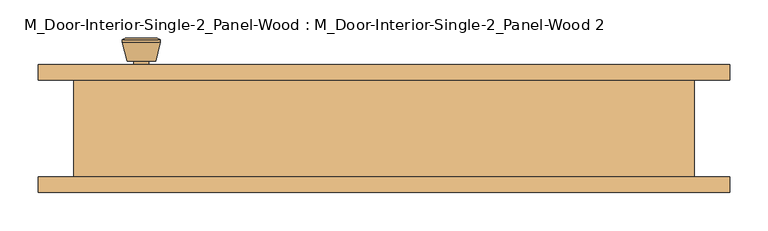
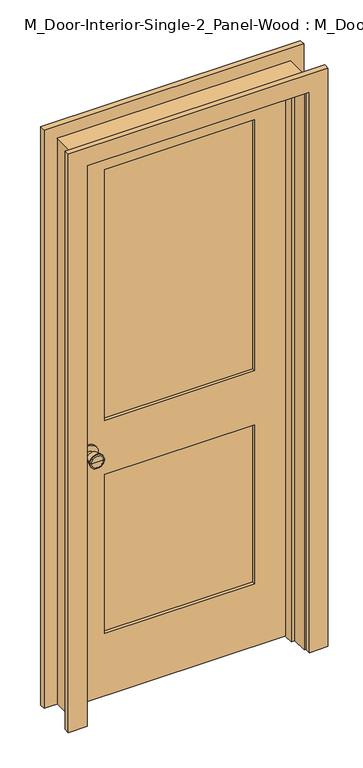
"""IFC4 building model written with IfcOpenShell, lengths in millimetres: door geometry, M_Door-Interior-Single-2_Panel-Wood : M_Door-Interior-Single-2_Panel-Wood 2."""

from ifc_helpers import new_model, si_unit, point, frame, frame_2d, origin, place, context, project, spatial, polyline, circle_curve, trimmed, segment, composite_curve, outline, extrude, faceted_brep, source, transform, mapped, element, save
from ifc_brep_helpers import plane_surface, cylinder_surface, revolved_surface, advanced_brep


def m_door_interior_single_2_panel_wood_m_door_interior_single_2_3351e8e6(model_context):
    return source(origin(), model_context, "Body", "SolidModel", [
        advanced_brep(
        [(-317.5, 19.325, 914.4), (-307.5, 19.325, 914.4), (-327.5, 19.325, 914.4), (-297.0241324, -29.675, 914.4), (-317.5, -29.675, 914.4), (-337.9758676, -29.675, 914.4), (-292.5, -27.8471319, 914.4), (-342.5, -27.8471319, 914.4), (-292.5, -24.3834537, 914.4), (-342.5, -24.3834537, 914.4), (-298.863764, 0.325, 914.4), (-336.136236, 0.325, 914.4), (-307.5, 0.325, 914.4), (-327.5, 0.325, 914.4)],
        [
            (0, 1),
            (1, 2, circle_curve(frame((-317.5, 19.325, 914.4), z_axis=(0.0, 1.0, 0.0), x_axis=(-1.0, 0.0, 0.0)), 10.0)),
            (2, 0),
            (2, 1, circle_curve(frame((-317.5, 19.325, 914.4), z_axis=(0.0, 1.0, 0.0), x_axis=(-1.0, 0.0, 0.0)), 10.0)),
            (3, 4),
            (4, 5),
            (5, 3, circle_curve(frame((-317.5, -29.675, 914.4), z_axis=(0.0, -1.0, 0.0), x_axis=(-1.0, 0.0, 0.0)), 20.4758676)),
            (3, 5, circle_curve(frame((-317.5, -29.675, 914.4), z_axis=(0.0, -1.0, 0.0), x_axis=(-1.0, 0.0, 0.0)), 20.4758676)),
            (6, 3),
            (5, 7),
            (7, 6, circle_curve(frame((-317.5, -27.8471319, 914.4), z_axis=(0.0, -1.0, 0.0), x_axis=(-1.0, 0.0, 0.0)), 25.0)),
            (6, 7, circle_curve(frame((-317.5, -27.8471319, 914.4), z_axis=(0.0, -1.0, 0.0), x_axis=(-1.0, 0.0, 0.0)), 25.0)),
            (8, 6),
            (7, 9),
            (9, 8, circle_curve(frame((-317.5, -24.3834537, 914.4), z_axis=(0.0, -1.0, 0.0), x_axis=(-1.0, 0.0, 0.0)), 25.0)),
            (8, 9, circle_curve(frame((-317.5, -24.3834537, 914.4), z_axis=(0.0, -1.0, 0.0), x_axis=(-1.0, 0.0, 0.0)), 25.0)),
            (10, 8),
            (9, 11),
            (11, 10, circle_curve(frame((-317.5, 0.325, 914.4), z_axis=(0.0, -1.0, 0.0), x_axis=(-1.0, 0.0, 0.0)), 18.636236)),
            (10, 11, circle_curve(frame((-317.5, 0.325, 914.4), z_axis=(0.0, -1.0, 0.0), x_axis=(-1.0, 0.0, 0.0)), 18.636236)),
            (12, 10),
            (11, 13),
            (13, 12, circle_curve(frame((-317.5, 0.325, 914.4), z_axis=(0.0, -1.0, 0.0), x_axis=(-1.0, 0.0, 0.0)), 10.0)),
            (12, 13, circle_curve(frame((-317.5, 0.325, 914.4), z_axis=(0.0, -1.0, 0.0), x_axis=(-1.0, 0.0, 0.0)), 10.0)),
            (1, 12),
            (13, 2),
        ],
        [
            plane_surface(frame((-317.5, 19.325, 914.4), z_axis=(0.0, 1.0, 0.0), x_axis=(-1.0, 0.0, 0.0))),
            plane_surface(frame((-317.5, -29.675, 914.4), z_axis=(0.0, -1.0, 0.0), x_axis=(-1.0, 0.0, 0.0))),
            revolved_surface(polyline([(-337.9758676, -29.675, 914.4), (-342.5, -27.8471319, 914.4)]), (-317.5, 19.325, 914.4), (0.0, 1.0, 0.0)),
            cylinder_surface(frame((-317.5, 19.325, 914.4), z_axis=(0.0, 1.0, 0.0), x_axis=(-1.0, 0.0, 0.0)), 25.0),
            revolved_surface(polyline([(-342.5, -24.3834537, 914.4), (-336.136236, 0.325, 914.4)]), (-317.5, 19.325, 914.4), (0.0, 1.0, 0.0)),
            plane_surface(frame((-317.5, 0.325, 914.4), z_axis=(0.0, 1.0, 0.0), x_axis=(-1.0, 0.0, 0.0))),
            cylinder_surface(frame((-317.5, 19.325, 914.4), z_axis=(0.0, 1.0, 0.0), x_axis=(-1.0, 0.0, 0.0)), 10.0),
        ],
        [
            (0, [[1, 2, 3]]),
            (0, [[-3, 4, -1]]),
            (1, [[5, 6, 7]]),
            (1, [[-6, -5, 8]]),
            (2, [[9, -7, 10, 11]]),
            (2, [[-10, -8, -9, 12]]),
            (3, [[13, -11, 14, 15]]),
            (3, [[-14, -12, -13, 16]]),
            (4, [[17, -15, 18, 19]]),
            (4, [[-18, -16, -17, 20]]),
            (5, [[21, -19, 22, 23]]),
            (5, [[-22, -20, -21, 24]]),
            (6, [[25, -23, 26, -2]]),
            (6, [[-26, -24, -25, -4]]),
        ],
    ),
        extrude(outline(composite_curve([segment(trimmed(circle_curve(frame_2d((914.4, -317.5)), 30.0), [point((914.4, -347.5))], [point((914.4, -287.5))], False, "CARTESIAN"), True, "CONTINUOUS"), segment(trimmed(circle_curve(frame_2d((914.4, -317.5)), 30.0), [point((914.4, -287.5))], [point((914.4, -347.5))], False, "CARTESIAN"), True, "CONTINUOUS")], self_intersect=False)), frame((0.0, 19.325, 0.0), z_axis=(0.0, 1.0, 0.0), x_axis=(0.0, 0.0, 1.0)), (0.0, 0.0, 1.0), 6.0),
        advanced_brep(
        [(-317.5, 66.325, 914.4), (-327.5, 66.325, 914.4), (-307.5, 66.325, 914.4), (-297.0241324, 115.325, 914.4), (-337.9758676, 115.325, 914.4), (-317.5, 115.325, 914.4), (-292.5, 113.4971319, 914.4), (-342.5, 113.4971319, 914.4), (-292.5, 110.0334537, 914.4), (-342.5, 110.0334537, 914.4), (-298.863764, 85.325, 914.4), (-336.136236, 85.325, 914.4), (-307.5, 85.325, 914.4), (-327.5, 85.325, 914.4)],
        [
            (0, 1),
            (1, 2, circle_curve(frame((-317.5, 66.325, 914.4), z_axis=(0.0, -1.0, 0.0), x_axis=(-1.0, 0.0, 0.0)), 10.0)),
            (2, 0),
            (2, 1, circle_curve(frame((-317.5, 66.325, 914.4), z_axis=(0.0, -1.0, 0.0), x_axis=(-1.0, 0.0, 0.0)), 10.0)),
            (3, 4, circle_curve(frame((-317.5, 115.325, 914.4), z_axis=(0.0, 1.0, 0.0), x_axis=(-1.0, 0.0, 0.0)), 20.4758676)),
            (4, 5),
            (5, 3),
            (4, 3, circle_curve(frame((-317.5, 115.325, 914.4), z_axis=(0.0, 1.0, 0.0), x_axis=(-1.0, 0.0, 0.0)), 20.4758676)),
            (6, 7, circle_curve(frame((-317.5, 113.4971319, 914.4), z_axis=(0.0, 1.0, 0.0), x_axis=(-1.0, 0.0, 0.0)), 25.0)),
            (7, 4),
            (3, 6),
            (7, 6, circle_curve(frame((-317.5, 113.4971319, 914.4), z_axis=(0.0, 1.0, 0.0), x_axis=(-1.0, 0.0, 0.0)), 25.0)),
            (8, 9, circle_curve(frame((-317.5, 110.0334537, 914.4), z_axis=(0.0, 1.0, 0.0), x_axis=(-1.0, 0.0, 0.0)), 25.0)),
            (9, 7),
            (6, 8),
            (9, 8, circle_curve(frame((-317.5, 110.0334537, 914.4), z_axis=(0.0, 1.0, 0.0), x_axis=(-1.0, 0.0, 0.0)), 25.0)),
            (10, 11, circle_curve(frame((-317.5, 85.325, 914.4), z_axis=(0.0, 1.0, 0.0), x_axis=(-1.0, 0.0, 0.0)), 18.636236)),
            (11, 9),
            (8, 10),
            (11, 10, circle_curve(frame((-317.5, 85.325, 914.4), z_axis=(0.0, 1.0, 0.0), x_axis=(-1.0, 0.0, 0.0)), 18.636236)),
            (12, 13, circle_curve(frame((-317.5, 85.325, 914.4), z_axis=(0.0, 1.0, 0.0), x_axis=(-1.0, 0.0, 0.0)), 10.0)),
            (13, 11),
            (10, 12),
            (13, 12, circle_curve(frame((-317.5, 85.325, 914.4), z_axis=(0.0, 1.0, 0.0), x_axis=(-1.0, 0.0, 0.0)), 10.0)),
            (1, 13),
            (12, 2),
        ],
        [
            plane_surface(frame((-317.5, 66.325, 914.4), z_axis=(0.0, -1.0, 0.0), x_axis=(-1.0, 0.0, 0.0))),
            plane_surface(frame((-317.5, 115.325, 914.4), z_axis=(0.0, 1.0, 0.0), x_axis=(-1.0, 0.0, 0.0))),
            revolved_surface(polyline([(-337.9758676, 115.325, 914.4), (-342.5, 113.4971319, 914.4)]), (-317.5, 66.325, 914.4), (0.0, -1.0, 0.0)),
            cylinder_surface(frame((-317.5, 66.325, 914.4), z_axis=(0.0, -1.0, 0.0), x_axis=(-1.0, 0.0, 0.0)), 25.0),
            revolved_surface(polyline([(-342.5, 110.0334537, 914.4), (-336.136236, 85.325, 914.4)]), (-317.5, 66.325, 914.4), (0.0, -1.0, 0.0)),
            plane_surface(frame((-317.5, 85.325, 914.4), z_axis=(0.0, -1.0, 0.0), x_axis=(-1.0, 0.0, 0.0))),
            cylinder_surface(frame((-317.5, 66.325, 914.4), z_axis=(0.0, -1.0, 0.0), x_axis=(-1.0, 0.0, 0.0)), 10.0),
        ],
        [
            (0, [[1, 2, 3]]),
            (0, [[-3, 4, -1]]),
            (1, [[5, 6, 7]]),
            (1, [[8, -7, -6]]),
            (2, [[9, 10, -5, 11]]),
            (2, [[12, -11, -8, -10]]),
            (3, [[13, 14, -9, 15]]),
            (3, [[16, -15, -12, -14]]),
            (4, [[17, 18, -13, 19]]),
            (4, [[20, -19, -16, -18]]),
            (5, [[21, 22, -17, 23]]),
            (5, [[24, -23, -20, -22]]),
            (6, [[-2, 25, -21, 26]]),
            (6, [[-4, -26, -24, -25]]),
        ],
    ),
        extrude(outline(composite_curve([segment(trimmed(circle_curve(frame_2d((914.4, -317.5)), 30.0), [point((914.4, -347.5))], [point((914.4, -287.5))], False, "CARTESIAN"), True, "CONTINUOUS"), segment(trimmed(circle_curve(frame_2d((914.4, -317.5)), 30.0), [point((914.4, -287.5))], [point((914.4, -347.5))], False, "CARTESIAN"), True, "CONTINUOUS")], self_intersect=False)), frame((0.0, 60.325, 0.0), z_axis=(0.0, 1.0, 0.0), x_axis=(0.0, 0.0, 1.0)), (0.0, 0.0, 1.0), 6.0),
        extrude(outline(polyline([(261.0, 36.9916667), (-261.0, 36.9916667), (-261.0, 48.6583333), (261.0, 48.6583333), (261.0, 36.9916667)])), frame((0.0, 0.0, 1014.4), z_axis=(0.0, 0.0, 1.0), x_axis=(1.0, 0.0, 0.0)), (0.0, 0.0, 1.0), 923.0),
        extrude(outline(polyline([(261.0, 36.9916667), (-261.0, 36.9916667), (-261.0, 48.6583333), (261.0, 48.6583333), (261.0, 36.9916667)])), frame((0.0, 0.0, 230.0), z_axis=(0.0, 0.0, 1.0), x_axis=(1.0, 0.0, 0.0)), (0.0, 0.0, 1.0), 584.4),
        extrude(outline(polyline([(2057.4, -381.0), (0.0, -381.0), (0.0, 381.0), (2057.4, 381.0), (2057.4, -381.0)]), holes=[polyline([(1937.4, -261.0), (1937.4, 261.0), (1014.4, 261.0), (1014.4, -261.0), (1937.4, -261.0)]), polyline([(814.4, -261.0), (814.4, 261.0), (230.0, 261.0), (230.0, -261.0), (814.4, -261.0)])]), frame((0.0, 25.325, 0.0), z_axis=(0.0, 1.0, 0.0), x_axis=(0.0, 0.0, 1.0)), (0.0, 0.0, 1.0), 35.0),
        faceted_brep([(406.0, 60.325, 0.0), (406.0, -66.675, 0.0), (381.0, -66.675, 0.0), (381.0, -9.6, 0.0), (368.3, -9.6, 0.0), (368.3, 25.325, 0.0), (381.0, 25.325, 0.0), (381.0, 60.325, 0.0), (406.0, 60.325, 2082.4), (406.0, -66.675, 2082.4), (-406.0, -66.675, 2082.4), (-406.0, -66.675, 0.0), (-381.0, -66.675, 0.0), (-381.0, -66.675, 2057.4), (381.0, -66.675, 2057.4), (381.0, -9.6, 2057.4), (-381.0, -9.6, 2057.4), (-381.0, -9.6, 0.0), (-368.3, -9.6, 0.0), (-368.3, -9.6, 2044.7), (368.3, -9.6, 2044.7), (368.3, 25.325, 2044.7), (-368.3, 25.325, 2044.7), (-368.3, 25.325, 0.0), (-381.0, 25.325, 0.0), (-381.0, 25.325, 2057.4), (381.0, 25.325, 2057.4), (381.0, 60.325, 2057.4), (-381.0, 60.325, 2057.4), (-381.0, 60.325, 0.0), (-406.0, 60.325, 0.0), (-406.0, 60.325, 2082.4)], [[[0, 1, 2, 3, 4, 5, 6, 7]], [[1, 0, 8, 9]], [[2, 1, 9, 10, 11, 12, 13, 14]], [[3, 2, 14, 15]], [[4, 3, 15, 16, 17, 18, 19, 20]], [[5, 4, 20, 21]], [[6, 5, 21, 22, 23, 24, 25, 26]], [[7, 6, 26, 27]], [[0, 7, 27, 28, 29, 30, 31, 8]], [[9, 8, 31, 10]], [[15, 14, 13, 16]], [[21, 20, 19, 22]], [[27, 26, 25, 28]], [[30, 29, 24, 23, 18, 17, 12, 11]], [[10, 31, 30, 11]], [[16, 13, 12, 17]], [[22, 19, 18, 23]], [[28, 25, 24, 29]]]),
        extrude(outline(polyline([(0.0, 387.35), (0.0, 452.35), (2128.75, 452.35), (2128.75, -452.35), (0.0, -452.35), (0.0, -387.35), (2063.75, -387.35), (2063.75, 387.35), (0.0, 387.35)])), frame((0.0, -86.675, 0.0), z_axis=(0.0, 1.0, 0.0), x_axis=(0.0, 0.0, 1.0)), (0.0, 0.0, 1.0), 20.0),
        extrude(outline(polyline([(0.0, 387.35), (0.0, 452.35), (2128.75, 452.35), (2128.75, -452.35), (0.0, -452.35), (0.0, -387.35), (2063.75, -387.35), (2063.75, 387.35), (0.0, 387.35)])), frame((0.0, 60.325, 0.0), z_axis=(0.0, 1.0, 0.0), x_axis=(0.0, 0.0, 1.0)), (0.0, 0.0, 1.0), 20.0),
    ])


if __name__ == "__main__":
    model = new_model("IFC4")
    model_context = context("Model", 3, world=origin())
    ifc_project = project(units=[si_unit("LENGTHUNIT", "METRE", prefix="MILLI")], contexts=[model_context])
    site = spatial("IfcSite", under=ifc_project)
    building = spatial("IfcBuilding", under=site)
    placement = place(None, origin())
    m_door_interior_single_2_panel_wood_m_door_interior_single_2_shape = m_door_interior_single_2_panel_wood_m_door_interior_single_2_3351e8e6(model_context)
    element("IfcDoor", 1, ObjectType="M_Door-Interior-Single-2_Panel-Wood : M_Door-Interior-Single-2_Panel-Wood 2", at=placement, inside=building, context=model_context, shape_type="MappedRepresentation", body=[
        mapped(m_door_interior_single_2_panel_wood_m_door_interior_single_2_shape, transform((0.0, 0.0, 0.0), x_axis=(1.0, 0.0, 0.0), y_axis=(0.0, 1.0, 0.0), z_axis=(0.0, 0.0, 1.0))),
    ])
    save(model, "model.ifc")

# Revit data of these elements
# Type "M_Door-Interior-Single-2_Panel-Wood : M_Door-Interior-Single-2_Panel-Wood 2"
#   Type Mark = "j"
#   Assembly Code = "C1020300"
#   Analytic Construction = "Wooden"
#   Top Rail = 0' - 4.72441"
#   Thickness = 0' - 1.37795"
#   Thermal Resistance (R) = 0.455703 (m²·K)/W
#   Swing Angle [instance default] = 90.00°
#   Stiles = 0' - 4.72441"
#   Rough Width = 2' - 7.9685"
#   Rough Height = 6' - 9.98425"
#   Lock Rail = 0' - 7.87402"
#   Height = 6' - 9"
#   Width = 2' - 6"
#   Heat Transfer Coefficient (U) = 2.19465 W/(m²·K)
#   Bottom Rail = 0' - 9.05512"
#   Trim Material = Cherry
#   Panel Material = Cherry
#   Frame Material = Cherry
#   Door Handle Material = Aluminum
#   Visual Light Transmittance = 0
#   Solar Heat Gain Coefficient = 0
#   Wall Closure = (empty or 0)
#   Function = (empty or 0)
# Element 1 (IfcDoor, "M_Door-Interior-Single-2_Panel-Wood : M_Door-Interior-Single-2_Panel-Wood 2")
#   Materials on its faces: "Cherry", "Aluminum"
# Materials
#   "Cherry": class "Wood", colour RGB 154 107 61, transparency 0, Description = "Prunus Serotina", Cost = 0
#   "Aluminum": class "Metal", colour RGB 244 244 244, transparency 0, Description = "Aluminum 6061", Cost = 0
